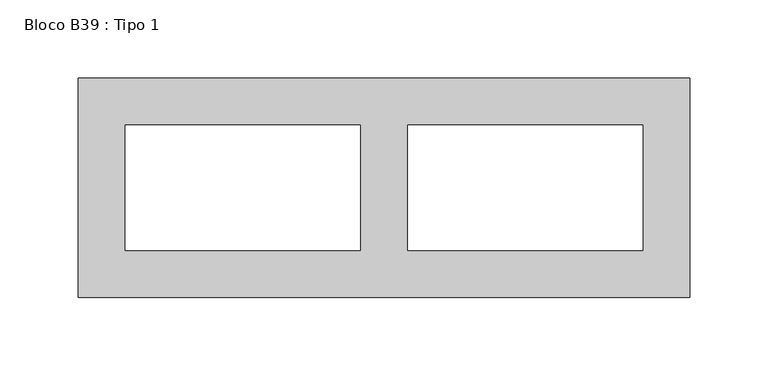
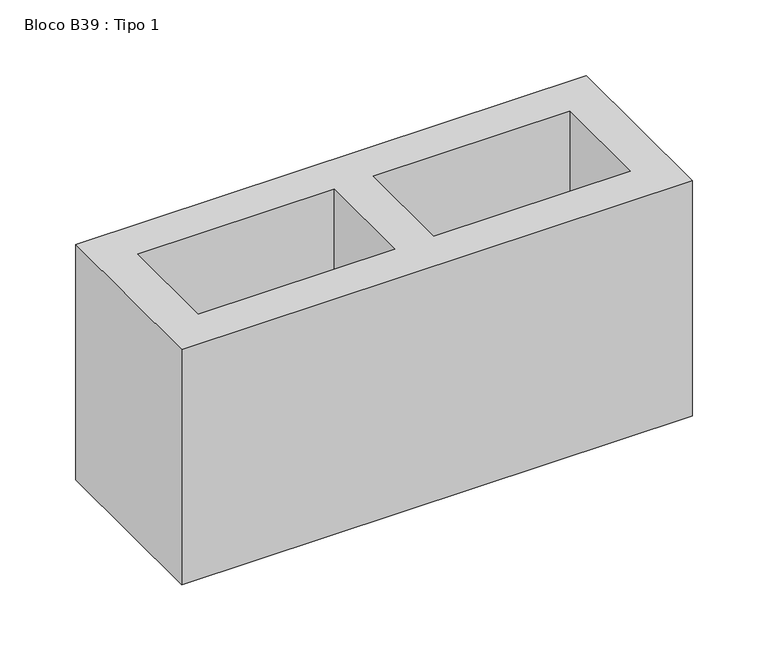
"""IFC4 building model written with IfcOpenShell, lengths in millimetres: proxy geometry, Bloco B39 : Tipo 1."""

from ifc_helpers import new_model, si_unit, origin, origin_with_axes, place, context, project, spatial, polyline, outline, extrude, source, transform, mapped, element, save


def bloco_b39_tipo_1_0929dc7b(model_context):
    return source(origin(), model_context, "Body", "SweptSolid", [
        extrude(outline(polyline([(390.0, 140.0), (390.0, 0.0), (0.0, 0.0), (0.0, 140.0), (390.0, 140.0)]), holes=[polyline([(180.0, 110.0), (30.0, 110.0), (30.0, 30.0), (180.0, 30.0), (180.0, 110.0)]), polyline([(210.0, 110.0), (210.0, 30.0), (360.0, 30.0), (360.0, 110.0), (210.0, 110.0)])]), origin_with_axes(), (0.0, 0.0, 1.0), 190.0),
    ])


if __name__ == "__main__":
    model = new_model("IFC4")
    model_context = context("Model", 3, world=origin())
    ifc_project = project(units=[si_unit("LENGTHUNIT", "METRE", prefix="MILLI")], contexts=[model_context])
    site = spatial("IfcSite", under=ifc_project)
    building = spatial("IfcBuilding", under=site)
    placement = place(None, origin())
    bloco_b39_tipo_1_shape = bloco_b39_tipo_1_0929dc7b(model_context)
    element("IfcBuildingElementProxy", 1, Name="Bloco B39 : Tipo 1", ObjectType="Bloco B39 : Tipo 1", at=placement, inside=building, context=model_context, shape_type="MappedRepresentation", body=[
        mapped(bloco_b39_tipo_1_shape, transform((0.0, 0.0, 0.0), x_axis=(1.0, 0.0, 0.0), y_axis=(0.0, 1.0, 0.0), z_axis=(0.0, 0.0, 1.0))),
    ])
    save(model, "model.ifc")

# Revit data of these elements
# Project information
#   built-in parameter 1006321 = "01/01/2010"
#   built-in parameter 1006320 = "GDPProjetos.RVT"
#   built-in parameter 1006319 = "RAQUEL CANELLAS"
#   built-in parameter 1006318 = "Av. Treze de Maio 13 sl.1414  |Centro | Rio de Janeiro"
#   built-in parameter 1006317 = "GDP - Gerenciamento e Desenvolvimento de Projetos"
#   built-in parameter 1006316 = "100"
# Type "Bloco B39 : Tipo 1"
#   SINAPI = ""
#   Assembly Code = ""
